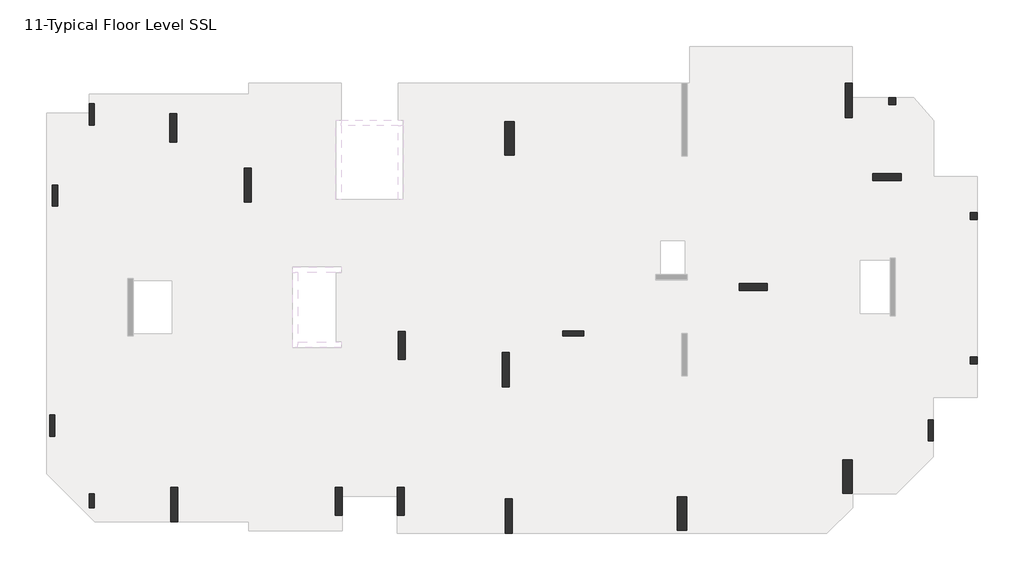
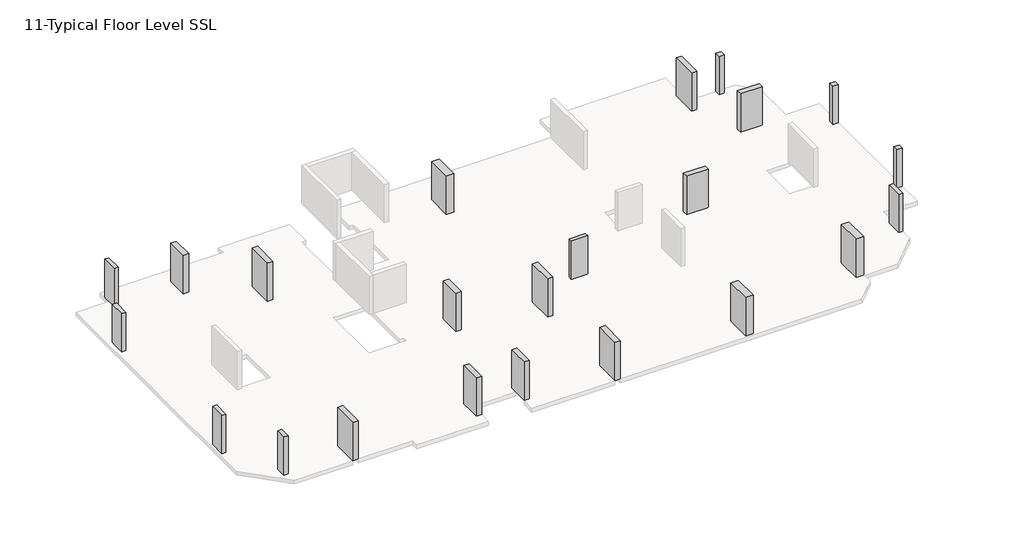
# One storey, part 2 of 2: 23 columns.
"""IFC4 building model written with IfcOpenShell, lengths in millimetres."""

import ifcopenshell
import ifcopenshell.guid

model = None  # the IFC model being written
_history = None  # IfcOwnerHistory: only IFC2X3 demands one
_inside = {}  # id of a spatial element -> (the spatial element, [elements in it])
_under = {}  # id of a project, library or spatial element -> (it, [spatial elements below it])
_declared = {}  # id of a project -> (the project, [libraries it declares])
_typed = {}  # id of a type object -> (the type object, [elements of that type])
_made_of = {}  # id of a material, layer set ... -> (it, [elements and type objects made of it])


def new_model(schema):
    """Start an empty IFC model of exactly this schema.

    Asked for "IFC4X3", IfcOpenShell would pick the latest addendum, in which some entities
    have other attributes; the version numbers below select the first issue.
    IFC2X3 requires an IfcOwnerHistory on every rooted entity: one is made here for all.
    """
    global model, _history
    if schema == "IFC4X3":
        model = ifcopenshell.file(schema_version=(4, 3, 0, 0))
    else:
        model = ifcopenshell.file(schema=schema)
    _inside.clear()
    _under.clear()
    _declared.clear()
    _typed.clear()
    _made_of.clear()
    _history = None
    if model.schema == "IFC2X3":
        org = make("IfcOrganization", Name="unknown")
        user = make(
            "IfcPersonAndOrganization",
            ThePerson=make("IfcPerson", FamilyName="unknown"),
            TheOrganization=org,
        )
        app = make(
            "IfcApplication",
            ApplicationDeveloper=org,
            Version="unknown",
            ApplicationFullName="unknown",
            ApplicationIdentifier="unknown",
        )
        _history = make(
            "IfcOwnerHistory",
            OwningUser=user,
            OwningApplication=app,
            ChangeAction="ADDED",
            CreationDate=0,
        )
    return model


def make(cls, **values):
    """One entity of the class cls with the attributes given. An attribute that is None is left unset."""
    return model.create_entity(
        cls, **{name: value for name, value in values.items() if value is not None}
    )


def rooted(cls, **values):
    """An entity with a GlobalId (a new one), such as an element, a storey or a relation."""
    return make(cls, GlobalId=ifcopenshell.guid.new(), OwnerHistory=_history, **values)


def si_unit(unit_type, name, prefix=None):
    """IfcSIUnit, for example si_unit("LENGTHUNIT", "METRE", prefix="MILLI")."""
    return make("IfcSIUnit", UnitType=unit_type, Prefix=prefix, Name=name)


def assignment(units):
    """IfcUnitAssignment: the units of a project."""
    return None if units is None else make("IfcUnitAssignment", Units=units)


def point(xyz):
    """IfcCartesianPoint."""
    return None if xyz is None else make("IfcCartesianPoint", Coordinates=xyz)


def direction(xyz):
    """IfcDirection."""
    return None if xyz is None else make("IfcDirection", DirectionRatios=xyz)


def frame(location, z_axis=None, x_axis=None):
    """IfcAxis2Placement3D, a coordinate frame: its origin and axes. An axis left out is left unset."""
    return make(
        "IfcAxis2Placement3D",
        Location=point(location),
        Axis=direction(z_axis),
        RefDirection=direction(x_axis),
    )


def origin():
    """The frame at (0, 0, 0) with its axes left unset."""
    return frame((0.0, 0.0, 0.0))


def place(relative_to, where):
    """IfcLocalPlacement: puts the frame where relative to a parent placement (None: the world)."""
    return make(
        "IfcLocalPlacement", PlacementRelTo=relative_to, RelativePlacement=where
    )


def context(
    kind, dimensions, precision=None, world=None, true_north=None, identifier=None
):
    """IfcGeometricRepresentationContext, for example the 3D "Model" context."""
    return make(
        "IfcGeometricRepresentationContext",
        ContextIdentifier=identifier,
        ContextType=kind,
        CoordinateSpaceDimension=dimensions,
        Precision=precision,
        WorldCoordinateSystem=world,
        TrueNorth=true_north,
    )


def project(units=None, contexts=None):
    """IfcProject with its units and contexts."""
    return rooted(
        "IfcProject",
        Name="project",
        RepresentationContexts=contexts,
        UnitsInContext=assignment(units),
    )


def spatial(cls, under=None, at=None, **own):
    """A site, building, storey or space (cls), placed at a placement, below another one or the project."""
    s = rooted(cls, ObjectPlacement=at, **own)
    if under is not None:
        _under.setdefault(under.id(), (under, []))[1].append(s)
    return s


def faces_of(points, faces, orient=None, outer=None):
    """IfcFace entities. A face is a list of loops; a loop is a list of indices into points, from 0.

    orient and outer hold one flag for each loop. By default every Orientation is true, the
    first loop of a face is its IfcFaceOuterBound and the others are IfcFaceBound.
    """
    made = []
    for i, loops in enumerate(faces):
        bounds = []
        for j, loop in enumerate(loops):
            is_outer = j == 0 if outer is None else outer[i][j]
            bounds.append(
                make(
                    "IfcFaceOuterBound" if is_outer else "IfcFaceBound",
                    Bound=make("IfcPolyLoop", Polygon=[points[k] for k in loop]),
                    Orientation=True if orient is None else orient[i][j],
                )
            )
        made.append(make("IfcFace", Bounds=bounds))
    return made


def faceted_brep(points, faces, orient=None, outer=None, voids=None):
    """IfcFacetedBrep: a solid bounded by flat faces; with voids (closed shells), ...WithVoids."""
    shared = [point(p) for p in points]
    hull = make("IfcClosedShell", CfsFaces=faces_of(shared, faces, orient, outer))
    if voids is None:
        return make("IfcFacetedBrep", Outer=hull)
    return make(
        "IfcFacetedBrepWithVoids",
        Outer=hull,
        Voids=[
            make(cls, CfsFaces=faces_of(shared, fs, o, b)) for cls, fs, o, b in voids
        ],
    )


def shape(context_of_items, identifier, shape_type, items):
    """IfcShapeRepresentation: the items that make up one representation, for example the "Body"."""
    return make(
        "IfcShapeRepresentation",
        ContextOfItems=context_of_items,
        RepresentationIdentifier=identifier,
        RepresentationType=shape_type,
        Items=items,
    )


def made_of(thing, what):
    """Note that an element or type object is made of a material, layer set ...; save() writes the relation."""
    if what is not None:
        _made_of.setdefault(what.id(), (what, []))[1].append(thing)
    return thing


def element(
    cls,
    number,
    at=None,
    inside=None,
    cuts=None,
    type_object=None,
    material=None,
    context=None,
    identifier="Body",
    shape_type=None,
    held_by="IfcProductDefinitionShape",
    body=None,
    shapes=None,
    **own,
):
    """One element of the class cls, such as IfcWall. Its Tag is "e" and its number.

    at: its placement. inside: the storey or other place that contains it. cuts: it is an
    opening in that element (IfcRelVoidsElement). A single representation is given by context,
    identifier, shape_type and body (its items); several are given by shapes. held_by: the class
    of the entity that holds the representations. save() writes the other relations.
    """
    e = rooted(cls, Tag="e%d" % number, ObjectPlacement=at, **own)
    if body is not None:
        shapes = [shape(context, identifier, shape_type, body)]
    if shapes is not None:
        e.Representation = make(held_by, Representations=shapes)
    if inside is not None:
        _inside.setdefault(inside.id(), (inside, []))[1].append(e)
    if cuts is not None:
        rooted(
            "IfcRelVoidsElement", RelatingBuildingElement=cuts, RelatedOpeningElement=e
        )
    if type_object is not None:
        _typed.setdefault(type_object.id(), (type_object, []))[1].append(e)
    return made_of(e, material)


def aggregate(whole, parts):
    """IfcRelAggregates: a whole, such as a stair, and the parts it consists of."""
    return rooted("IfcRelAggregates", RelatingObject=whole, RelatedObjects=parts)


def save(model, path):
    """Write the relations noted so far, then the file.

    IfcRelAggregates (storeys below a building ...), IfcRelContainedInSpatialStructure (elements
    in a storey), IfcRelDefinesByType, IfcRelAssociatesMaterial and IfcRelDeclares: one each for
    every whole, place, type object, material and project.
    """
    for whole, parts in _under.values():
        aggregate(whole, parts)
    for where, things in _inside.values():
        rooted(
            "IfcRelContainedInSpatialStructure",
            RelatedElements=things,
            RelatingStructure=where,
        )
    for kind, things in _typed.values():
        rooted("IfcRelDefinesByType", RelatedObjects=things, RelatingType=kind)
    for what, things in _made_of.values():
        rooted("IfcRelAssociatesMaterial", RelatedObjects=things, RelatingMaterial=what)
    for by, libraries in _declared.values():
        rooted("IfcRelDeclares", RelatingContext=by, RelatedDefinitions=libraries)
    model.write(path)


model = new_model("IFC4")

# Units and contexts
model_context = context("Model", 3, world=origin())
ifc_project = project(units=[si_unit("LENGTHUNIT", "METRE", prefix="MILLI")], contexts=[model_context])

# Site, building, storey
site = spatial("IfcSite", under=ifc_project)
building = spatial("IfcBuilding", under=site)
storey = spatial("IfcBuildingStorey", under=building, Name="11-Typical Floor Level SSL", Elevation=27000.0)

# Columns
placement = place(None, origin())
element("IfcColumn", 1, ObjectType="M_Concrete-Rectangular-Column : C-1 (400 x 400mm)", at=placement, inside=storey, context=model_context, shape_type="Brep", body=[
    faceted_brep([(52549.9999998, 16712.0, 27000.0), (52549.9999998, 16312.0, 27000.0), (52149.9999998, 16312.0, 27000.0), (52149.9999998, 16712.0, 27000.0), (52549.9999998, 16712.0, 30000.0), (52549.9999998, 16312.0, 30000.0), (52549.9999998, 16312.0, 29700.0), (52549.9999998, 16712.0, 29700.0), (52149.9999998, 16312.0, 30000.0), (52149.9999998, 16312.0, 29700.0), (52149.9999998, 16712.0, 30000.0), (52149.9999998, 16712.0, 29700.0)], [[[0, 1, 2, 3]], [[4, 5, 6, 1, 0, 7]], [[5, 8, 9, 2, 1, 6]], [[8, 10, 11, 3, 2, 9]], [[10, 4, 7, 0, 3, 11]], [[4, 10, 8, 5]]]),
])
element("IfcColumn", 2, ObjectType="M_Concrete-Rectangular-Column : C-1 (400 x 400mm)", at=placement, inside=storey, context=model_context, shape_type="Brep", body=[
    faceted_brep([(47898.6337868, 23252.0, 27000.0), (47898.6337868, 22852.0, 27000.0), (47498.6337868, 22852.0, 27000.0), (47498.6337868, 23252.0, 27000.0), (47898.6337868, 23252.0, 30000.0), (47898.6337868, 22852.0, 30000.0), (47898.6337868, 22852.0, 29700.0), (47498.6337868, 22852.0, 30000.0), (47498.6337868, 22852.0, 29700.0), (47498.6337868, 23252.0, 30000.0)], [[[0, 1, 2, 3]], [[4, 5, 6, 1, 0]], [[5, 7, 8, 2, 1, 6]], [[7, 9, 3, 2, 8]], [[9, 4, 0, 3]], [[4, 9, 7, 5]]]),
])
element("IfcColumn", 3, ObjectType="M_Concrete-Rectangular-Column : C-1 (400 x 400mm)", at=placement, inside=storey, context=model_context, shape_type="Brep", body=[
    faceted_brep([(52549.9999998, 8504.0039609, 27000.0), (52549.9999998, 8104.0039609, 27000.0), (52149.9999998, 8104.0039609, 27000.0), (52149.9999998, 8504.0039609, 27000.0), (52549.9999998, 8504.0039609, 30000.0), (52549.9999998, 8104.0039609, 30000.0), (52549.9999998, 8104.0039609, 29700.0), (52549.9999998, 8504.0039609, 29700.0), (52149.9999998, 8104.0039609, 30000.0), (52149.9999998, 8104.0039609, 29700.0), (52149.9999998, 8504.0039609, 30000.0), (52149.9999998, 8504.0039609, 29700.0)], [[[0, 1, 2, 3]], [[4, 5, 6, 1, 0, 7]], [[5, 8, 9, 2, 1, 6]], [[8, 10, 11, 3, 2, 9]], [[10, 4, 7, 0, 3, 11]], [[4, 10, 8, 5]]]),
])
element("IfcColumn", 4, ObjectType="M_Concrete-Rectangular-Column : C-2 (300 x 800mm)", at=placement, inside=storey, context=model_context, shape_type="Brep", body=[
    faceted_brep([(2352.0, 728.0, 27000.0), (2352.0, -72.0, 27000.0), (2052.0, -72.0, 27000.0), (2052.0, 728.0, 27000.0), (2352.0, 728.0, 30000.0), (2352.0, -72.0, 30000.0), (2352.0, -72.0, 29700.0), (2352.0, 728.0, 29700.0), (2052.0, -72.0, 30000.0), (2052.0, -72.0, 29700.0), (2052.0, 728.0, 30000.0), (2052.0, 728.0, 29700.0)], [[[0, 1, 2, 3]], [[4, 5, 6, 1, 0, 7]], [[5, 8, 9, 2, 1, 6]], [[8, 10, 11, 3, 2, 9]], [[10, 4, 7, 0, 3, 11]], [[4, 10, 8, 5]]]),
])
element("IfcColumn", 5, ObjectType="M_Concrete-Rectangular-Column : C-3(300 x 1200mm)", at=placement, inside=storey, context=model_context, shape_type="Brep", body=[
    faceted_brep([(2352.0, 22908.0000656, 27000.0), (2352.0, 21708.0000656, 27000.0), (2052.0, 21708.0000656, 27000.0), (2052.0, 22908.0000656, 27000.0), (2352.0, 22908.0000656, 30000.0), (2352.0, 21708.0000656, 30000.0), (2352.0, 21708.0000656, 29700.0), (2352.0, 22908.0000656, 29700.0), (2052.0, 21708.0000656, 30000.0), (2052.0, 21708.0000656, 29700.0), (2052.0, 22380.0004589, 30000.0), (2052.0, 22908.0000656, 30000.0), (2052.0, 22908.0000656, 29700.0)], [[[0, 1, 2, 3]], [[4, 5, 6, 1, 0, 7]], [[5, 8, 9, 2, 1, 6]], [[8, 10, 11, 12, 3, 2, 9]], [[11, 4, 7, 0, 3, 12]], [[4, 11, 10, 8, 5]]]),
])
element("IfcColumn", 6, ObjectType="M_Concrete-Rectangular-Column : C-3(300 x 1200mm)", at=placement, inside=storey, context=model_context, shape_type="Brep", body=[
    faceted_brep([(257.9999999, 18288.0, 27000.0), (257.9999999, 17088.0, 27000.0), (-42.0000001, 17088.0, 27000.0), (-42.0000001, 18288.0, 27000.0), (257.9999999, 18288.0, 30000.0), (257.9999999, 17088.0, 30000.0), (257.9999999, 17088.0, 29700.0), (257.9999999, 18288.0, 29700.0), (-42.0000001, 17088.0, 30000.0), (-42.0000001, 17088.0, 29700.0), (-42.0000001, 18288.0, 30000.0), (-42.0000001, 18288.0, 29700.0)], [[[0, 1, 2, 3]], [[4, 5, 6, 1, 0, 7]], [[5, 8, 9, 2, 1, 6]], [[8, 10, 11, 3, 2, 9]], [[10, 4, 7, 0, 3, 11]], [[4, 10, 8, 5]]]),
])
element("IfcColumn", 7, ObjectType="M_Concrete-Rectangular-Column : C-3(300 x 1200mm)", at=placement, inside=storey, context=model_context, shape_type="Brep", body=[
    faceted_brep([(108.001803, 5201.9999858, 27000.0), (108.001803, 4001.9999858, 27000.0), (-191.998197, 4001.9999858, 27000.0), (-191.998197, 5201.9999858, 27000.0), (108.001803, 5201.9999858, 30000.0), (108.001803, 4001.9999858, 30000.0), (108.001803, 4001.9999858, 29700.0), (108.001803, 5201.9999858, 29700.0), (-191.998197, 4001.9999858, 30000.0), (-191.998197, 4001.9999858, 29700.0), (-191.998197, 5201.9999858, 30000.0), (-191.998197, 5201.9999858, 29700.0)], [[[0, 1, 2, 3]], [[4, 5, 6, 1, 0, 7]], [[5, 8, 9, 2, 1, 6]], [[8, 10, 11, 3, 2, 9]], [[10, 4, 7, 0, 3, 11]], [[4, 10, 8, 5]]]),
])
element("IfcColumn", 8, ObjectType="M_Concrete-Rectangular-Column : C-3(300 x 1200mm)", at=placement, inside=storey, context=model_context, shape_type="Brep", body=[
    faceted_brep([(50046.0009271, 4931.9999929, 27000.0), (50046.0009271, 3731.9999929, 27000.0), (49746.0009271, 3731.9999929, 27000.0), (49746.0009271, 4931.9999929, 27000.0), (50046.0009271, 4931.9999929, 30000.0), (50046.0009271, 3731.9999929, 30000.0), (50046.0009271, 3731.9999929, 29700.0), (50046.0009271, 4931.9999929, 29700.0), (49746.0009271, 3731.9999929, 30000.0), (49746.0009271, 3731.9999929, 29700.0), (49746.0009271, 4931.9999929, 30000.0), (49746.0009271, 4931.9999929, 29700.0)], [[[0, 1, 2, 3]], [[4, 5, 6, 1, 0, 7]], [[5, 8, 9, 2, 1, 6]], [[8, 10, 11, 3, 2, 9]], [[10, 4, 7, 0, 3, 11]], [[4, 10, 8, 5]]]),
])
element("IfcColumn", 9, ObjectType="M_Concrete-Rectangular-Column : C-3(300 x 1200mm)", at=placement, inside=storey, context=model_context, shape_type="Brep", body=[
    faceted_brep([(28975.9999998, 9996.0000019, 27000.0), (30175.9999998, 9996.0000019, 27000.0), (30175.9999998, 9696.0000019, 27000.0), (28975.9999998, 9696.0000019, 27000.0), (28975.9999998, 9996.0000019, 30000.0), (30175.9999998, 9996.0000019, 30000.0), (30175.9999998, 9996.0000019, 29700.0), (28975.9999998, 9996.0000019, 29700.0), (30175.9999998, 9696.0000019, 30000.0), (30175.9999998, 9696.0000019, 29700.0), (28975.9999998, 9696.0000019, 30000.0), (28975.9999998, 9696.0000019, 29700.0)], [[[0, 1, 2, 3]], [[4, 5, 6, 1, 0, 7]], [[5, 8, 9, 2, 1, 6]], [[8, 10, 11, 3, 2, 9]], [[10, 4, 7, 0, 3, 11]], [[4, 10, 8, 5]]]),
])
element("IfcColumn", 10, ObjectType="M_Concrete-Rectangular-Column : C-4 (400 x 1600mm)", at=placement, inside=storey, context=model_context, shape_type="Brep", body=[
    faceted_brep([(7021.9999999, 22340.0000078, 27000.0), (7021.9999999, 20740.0000078, 27000.0), (6621.9999999, 20740.0000078, 27000.0), (6621.9999999, 22340.0000078, 27000.0), (7021.9999999, 22340.0000078, 30000.0), (7021.9999999, 20740.0000078, 30000.0), (7021.9999999, 20740.0000078, 29700.0), (7021.9999999, 22340.0000078, 29700.0), (6621.9999999, 20740.0000078, 30000.0), (6621.9999999, 20740.0000078, 29700.0), (6621.9999999, 22340.0000078, 30000.0), (6621.9999999, 22340.0000078, 29700.0)], [[[0, 1, 2, 3]], [[4, 5, 6, 1, 0, 7]], [[5, 8, 9, 2, 1, 6]], [[8, 10, 11, 3, 2, 9]], [[10, 4, 7, 0, 3, 11]], [[4, 10, 8, 5]]]),
])
element("IfcColumn", 11, ObjectType="M_Concrete-Rectangular-Column : C-4 (400 x 1600mm)", at=placement, inside=storey, context=model_context, shape_type="Brep", body=[
    faceted_brep([(19969.9997488, 1087.9955348, 27000.0), (19969.9997488, -512.0044652, 27000.0), (19569.9997488, -512.0044652, 27000.0), (19569.9997488, 1087.9955348, 27000.0), (19969.9997488, 1087.9955348, 30000.0), (19969.9997488, -512.0044652, 30000.0), (19969.9997488, -512.0044652, 29700.0), (19969.9997488, 1087.9955348, 29700.0), (19569.9997488, -512.0044652, 30000.0), (19569.9997488, -512.0044652, 29700.0), (19569.9997488, 564.000519, 30000.0), (19569.9997488, 1087.9955348, 30000.0), (19569.9997488, 1087.9955348, 29700.0)], [[[0, 1, 2, 3]], [[4, 5, 6, 1, 0, 7]], [[5, 8, 9, 2, 1, 6]], [[8, 10, 11, 12, 3, 2, 9]], [[11, 4, 7, 0, 3, 12]], [[4, 11, 10, 8, 5]]]),
])
element("IfcColumn", 12, ObjectType="M_Concrete-Rectangular-Column : C-4 (400 x 1600mm)", at=placement, inside=storey, context=model_context, shape_type="Brep", body=[
    faceted_brep([(46605.9993605, 18950.0, 27000.0), (48205.9993605, 18950.0, 27000.0), (48205.9993605, 18550.0, 27000.0), (46605.9993605, 18550.0, 27000.0), (46605.9993605, 18950.0, 30000.0), (48205.9993605, 18950.0, 30000.0), (48205.9993605, 18950.0, 29700.0), (46605.9993605, 18950.0, 29700.0), (48205.9993605, 18550.0, 30000.0), (48205.9993605, 18550.0, 29700.0), (46605.9993605, 18550.0, 30000.0), (46605.9993605, 18550.0, 29700.0)], [[[0, 1, 2, 3]], [[4, 5, 6, 1, 0, 7]], [[5, 8, 9, 2, 1, 6]], [[8, 10, 11, 3, 2, 9]], [[10, 4, 7, 0, 3, 11]], [[4, 10, 8, 5]]]),
])
element("IfcColumn", 13, ObjectType="M_Concrete-Rectangular-Column : C-5 (400 x 1600mm)", at=placement, inside=storey, context=model_context, shape_type="Brep", body=[
    faceted_brep([(20030.000009, 9955.9999979, 27000.0), (20030.000009, 8355.9999979, 27000.0), (19630.000009, 8355.9999979, 27000.0), (19630.000009, 9955.9999979, 27000.0), (20030.000009, 9955.9999979, 30000.0), (20030.000009, 8355.9999979, 30000.0), (20030.000009, 8355.9999979, 29700.0), (20030.000009, 9955.9999979, 29700.0), (19630.000009, 8355.9999979, 30000.0), (19630.000009, 8355.9999979, 29700.0), (19630.000009, 9955.9999979, 30000.0), (19630.000009, 9955.9999979, 29700.0)], [[[0, 1, 2, 3]], [[4, 5, 6, 1, 0, 7]], [[5, 8, 9, 2, 1, 6]], [[8, 10, 11, 3, 2, 9]], [[10, 4, 7, 0, 3, 11]], [[4, 10, 8, 5]]]),
])
element("IfcColumn", 14, ObjectType="M_Concrete-Rectangular-Column : C-5 (400 x 1600mm)", at=placement, inside=storey, context=model_context, shape_type="Brep", body=[
    faceted_brep([(16429.9999981, 1088.0, 27000.0), (16429.9999981, -512.0, 27000.0), (16029.9999981, -512.0, 27000.0), (16029.9999981, 1088.0, 27000.0), (16429.9999981, 1088.0, 30000.0), (16429.9999981, 564.000519, 30000.0), (16429.9999981, -512.0, 30000.0), (16429.9999981, -512.0, 29700.0), (16429.9999981, 1088.0, 29700.0), (16029.9999981, -512.0, 30000.0), (16029.9999981, -512.0, 29700.0), (16029.9999981, 1088.0, 30000.0), (16029.9999981, 1088.0, 29700.0)], [[[0, 1, 2, 3]], [[4, 5, 6, 7, 1, 0, 8]], [[6, 9, 10, 2, 1, 7]], [[9, 11, 12, 3, 2, 10]], [[11, 4, 8, 0, 3, 12]], [[4, 11, 9, 6, 5]]]),
])
element("IfcColumn", 15, ObjectType="M_Concrete-Rectangular-Column : C-5 (400 x 1600mm)", at=placement, inside=storey, context=model_context, shape_type="Brep", body=[
    faceted_brep([(38998.0014887, 12692.0079212, 27000.0), (40598.0014887, 12692.0079212, 27000.0), (40598.0014887, 12292.0079212, 27000.0), (38998.0014887, 12292.0079212, 27000.0), (38998.0014887, 12692.0079212, 30000.0), (40598.0014887, 12692.0079212, 30000.0), (40598.0014887, 12692.0079212, 29700.0), (38998.0014887, 12692.0079212, 29700.0), (40598.0014887, 12292.0079212, 30000.0), (40598.0014887, 12292.0079212, 29700.0), (38998.0014887, 12292.0079212, 30000.0), (38998.0014887, 12292.0079212, 29700.0)], [[[0, 1, 2, 3]], [[4, 5, 6, 1, 0, 7]], [[5, 8, 9, 2, 1, 6]], [[8, 10, 11, 3, 2, 9]], [[10, 4, 7, 0, 3, 11]], [[4, 10, 8, 5]]]),
])
element("IfcColumn", 16, ObjectType="M_Concrete-Rectangular-Column : C-6 (400 x 1950mm)", at=placement, inside=storey, context=model_context, shape_type="Brep", body=[
    faceted_brep([(11270.0000427, 19262.9999996, 27000.0), (11270.0000427, 17312.9999996, 27000.0), (10870.0000427, 17312.9999996, 27000.0), (10870.0000427, 19262.9999996, 27000.0), (11270.0000427, 19262.9999996, 30000.0), (11270.0000427, 17312.9999996, 30000.0), (11270.0000427, 17312.9999996, 29700.0), (11270.0000427, 19262.9999996, 29700.0), (10870.0000427, 17312.9999996, 30000.0), (10870.0000427, 17312.9999996, 29700.0), (10870.0000427, 19262.9999996, 30000.0), (10870.0000427, 19262.9999996, 29700.0)], [[[0, 1, 2, 3]], [[4, 5, 6, 1, 0, 7]], [[5, 8, 9, 2, 1, 6]], [[8, 10, 11, 3, 2, 9]], [[10, 4, 7, 0, 3, 11]], [[4, 10, 8, 5]]]),
])
element("IfcColumn", 17, ObjectType="M_Concrete-Rectangular-Column : C-6 (400 x 1950mm)", at=placement, inside=storey, context=model_context, shape_type="Brep", body=[
    faceted_brep([(7082.0000416, 1083.0000153, 27000.0), (7082.0000416, -866.9999847, 27000.0), (6682.0000416, -866.9999847, 27000.0), (6682.0000416, 1083.0000153, 27000.0), (7082.0000416, 1083.0000153, 30000.0), (7082.0000416, -866.9999847, 30000.0), (7082.0000416, -866.9999847, 29700.0), (7082.0000416, 1083.0000153, 29700.0), (6682.0000416, -866.9999847, 30000.0), (6682.0000416, -866.9999847, 29700.0), (6682.0000416, 1083.0000153, 30000.0), (6682.0000416, 1083.0000153, 29700.0)], [[[0, 1, 2, 3]], [[4, 5, 6, 1, 0, 7]], [[5, 8, 9, 2, 1, 6]], [[8, 10, 11, 3, 2, 9]], [[10, 4, 7, 0, 3, 11]], [[4, 10, 8, 5]]]),
])
element("IfcColumn", 18, ObjectType="M_Concrete-Rectangular-Column : C-6 (400 x 1950mm)", at=placement, inside=storey, context=model_context, shape_type="Brep", body=[
    faceted_brep([(26113.9999998, 422.995535, 27000.0), (26113.9999998, -1527.004465, 27000.0), (25713.9999998, -1527.004465, 27000.0), (25713.9999998, 422.995535, 27000.0), (26113.9999998, 422.995535, 30000.0), (26113.9999998, -1527.004465, 30000.0), (26113.9999998, -1527.004465, 29700.0), (26113.9999998, 422.995535, 29700.0), (25713.9999998, -1527.004465, 30000.0), (25713.9999998, -1527.004465, 29700.0), (25713.9999998, 422.995535, 30000.0), (25713.9999998, 422.995535, 29700.0)], [[[0, 1, 2, 3]], [[4, 5, 6, 1, 0, 7]], [[5, 8, 9, 2, 1, 6]], [[8, 10, 11, 3, 2, 9]], [[10, 4, 7, 0, 3, 11]], [[4, 10, 8, 5]]]),
])
element("IfcColumn", 19, ObjectType="M_Concrete-Rectangular-Column : C-6 (400 x 1950mm)", at=placement, inside=storey, context=model_context, shape_type="Brep", body=[
    faceted_brep([(45446.0007483, 24087.0, 27000.0), (45446.0007483, 22137.0, 27000.0), (45046.0007483, 22137.0, 27000.0), (45046.0007483, 24087.0, 27000.0), (45446.0007483, 24087.0, 30000.0), (45446.0007483, 23252.0000315, 30000.0), (45446.0007483, 22137.0, 30000.0), (45446.0007483, 22137.0, 29700.0), (45446.0007483, 24087.0, 29700.0), (45046.0007483, 22137.0, 30000.0), (45046.0007483, 22137.0, 29700.0), (45046.0007483, 24087.0, 30000.0), (45046.0007483, 24087.0, 29700.0)], [[[0, 1, 2, 3]], [[4, 5, 6, 7, 1, 0, 8]], [[6, 9, 10, 2, 1, 7]], [[9, 11, 12, 3, 2, 10]], [[11, 4, 8, 0, 3, 12]], [[4, 11, 9, 6, 5]]]),
])
element("IfcColumn", 20, ObjectType="M_Concrete-Rectangular-Column : C-6 (400 x 1950mm)", at=placement, inside=storey, context=model_context, shape_type="Brep", body=[
    faceted_brep([(25934.0000455, 8751.0001824, 27000.0), (25934.0000455, 6801.0001824, 27000.0), (25534.0000455, 6801.0001824, 27000.0), (25534.0000455, 8751.0001824, 27000.0), (25934.0000455, 8751.0001824, 30000.0), (25934.0000455, 6801.0001824, 30000.0), (25934.0000455, 6801.0001824, 29700.0), (25934.0000455, 8751.0001824, 29700.0), (25534.0000455, 6801.0001824, 30000.0), (25534.0000455, 6801.0001824, 29700.0), (25534.0000455, 8751.0001824, 30000.0), (25534.0000455, 8751.0001824, 29700.0)], [[[0, 1, 2, 3]], [[4, 5, 6, 1, 0, 7]], [[5, 8, 9, 2, 1, 6]], [[8, 10, 11, 3, 2, 9]], [[10, 4, 7, 0, 3, 11]], [[4, 10, 8, 5]]]),
])
element("IfcColumn", 21, ObjectType="M_Concrete-Rectangular-Column : C-7 (550 x 1900mm)", at=placement, inside=storey, context=model_context, shape_type="Brep", body=[
    faceted_brep([(36035.9999998, 548.0007983, 27000.0), (36035.9999998, -1351.9992017, 27000.0), (35485.9999998, -1351.9992017, 27000.0), (35485.9999998, 548.0007983, 27000.0), (36035.9999998, 548.0007983, 30000.0), (36035.9999998, -1351.9992017, 30000.0), (36035.9999998, -1351.9992017, 29700.0), (36035.9999998, 548.0007983, 29700.0), (35485.9999998, -1351.9992017, 30000.0), (35485.9999998, -1351.9992017, 29700.0), (35485.9999998, 548.0007983, 30000.0), (35485.9999998, 548.0007983, 29700.0)], [[[0, 1, 2, 3]], [[4, 5, 6, 1, 0, 7]], [[5, 8, 9, 2, 1, 6]], [[8, 10, 11, 3, 2, 9]], [[10, 4, 7, 0, 3, 11]], [[4, 10, 8, 5]]]),
])
element("IfcColumn", 22, ObjectType="M_Concrete-Rectangular-Column : C-7 (550 x 1900mm)", at=placement, inside=storey, context=model_context, shape_type="Brep", body=[
    faceted_brep([(45443.9999998, 2648.0, 27000.0), (45443.9999998, 748.0, 27000.0), (44893.9999998, 748.0, 27000.0), (44893.9999998, 2648.0, 27000.0), (45443.9999998, 2648.0, 30000.0), (45443.9999998, 748.0, 30000.0), (45443.9999998, 748.0, 29700.0), (45443.9999998, 2648.0, 29700.0), (44893.9999998, 748.0, 30000.0), (44893.9999998, 748.0, 29700.0), (44893.9999998, 2648.0, 30000.0), (44893.9999998, 2648.0, 29700.0)], [[[0, 1, 2, 3]], [[4, 5, 6, 1, 0, 7]], [[5, 8, 9, 2, 1, 6]], [[8, 10, 11, 3, 2, 9]], [[10, 4, 7, 0, 3, 11]], [[4, 10, 8, 5]]]),
])
element("IfcColumn", 23, ObjectType="M_Concrete-Rectangular-Column : C-7 (550 x 1900mm)", at=placement, inside=storey, context=model_context, shape_type="Brep", body=[
    faceted_brep([(26218.9999998, 21900.0, 27000.0), (26218.9999998, 20000.0, 27000.0), (25668.9999998, 20000.0, 27000.0), (25668.9999998, 21900.0, 27000.0), (26218.9999998, 21900.0, 30000.0), (26218.9999998, 20000.0, 30000.0), (26218.9999998, 20000.0, 29700.0), (26218.9999998, 21900.0, 29700.0), (25668.9999998, 20000.0, 30000.0), (25668.9999998, 20000.0, 29700.0), (25668.9999998, 21900.0, 30000.0), (25668.9999998, 21900.0, 29700.0)], [[[0, 1, 2, 3]], [[4, 5, 6, 1, 0, 7]], [[5, 8, 9, 2, 1, 6]], [[8, 10, 11, 3, 2, 9]], [[10, 4, 7, 0, 3, 11]], [[4, 10, 8, 5]]]),
])

save(model, "model.ifc")

# Revit data of these elements
# Type "M_Concrete-Rectangular-Column : C-1 (400 x 400mm)"
#   Type Mark = "C01"
#   b = 400 mm
#   h = 400 mm
#   Structural Material [instance default] = Concrete, Cast-in-Place gray
# Type "M_Concrete-Rectangular-Column : C-2 (300 x 800mm)"
#   Type Mark = "C02"
#   b = 300 mm
#   h = 800 mm
#   Structural Material [instance default] = Concrete, Cast-in-Place gray
# Type "M_Concrete-Rectangular-Column : C-3(300 x 1200mm)"
#   Type Mark = "C03"
#   b = 300 mm
#   h = 1200 mm
#   Structural Material [instance default] = Concrete, Cast-in-Place gray
# Type "M_Concrete-Rectangular-Column : C-4 (400 x 1600mm)"
#   Type Mark = "C04"
#   b = 400 mm
#   h = 1600 mm
#   Structural Material [instance default] = Concrete, Cast-in-Place gray
# Type "M_Concrete-Rectangular-Column : C-5 (400 x 1600mm)"
#   Type Mark = "C05"
#   b = 400 mm
#   h = 1600 mm
#   Structural Material [instance default] = Concrete, Cast-in-Place gray
# Type "M_Concrete-Rectangular-Column : C-6 (400 x 1950mm)"
#   Type Mark = "C06"
#   b = 400 mm
#   h = 1950 mm
#   Structural Material [instance default] = Concrete, Cast-in-Place gray
# Type "M_Concrete-Rectangular-Column : C-7 (550 x 1900mm)"
#   Type Mark = "C07"
#   b = 550 mm
#   h = 1900 mm
#   Structural Material [instance default] = Concrete, Cast-in-Place gray
# Elements 1, 2, 3 (IfcColumn, "M_Concrete-Rectangular-Column : C-1 (400 x 400mm)")
#   Structural Material = Concrete-RC
#   Phase Created = New Construction
#   Materials on its faces: "Concrete-RC"
# Element 4 (IfcColumn, "M_Concrete-Rectangular-Column : C-2 (300 x 800mm)")
#   Structural Material = Concrete-RC
#   Phase Created = New Construction
#   Materials on its faces: "Concrete-RC"
# Elements 5, 6, 7, 8, 9 (IfcColumn, "M_Concrete-Rectangular-Column : C-3(300 x 1200mm)")
#   Structural Material = Concrete-RC
#   Phase Created = New Construction
#   Materials on its faces: "Concrete-RC"
# Elements 10, 11, 12 (IfcColumn, "M_Concrete-Rectangular-Column : C-4 (400 x 1600mm)")
#   Structural Material = Concrete-RC
#   Phase Created = New Construction
#   Materials on its faces: "Concrete-RC"
# Elements 13, 14, 15 (IfcColumn, "M_Concrete-Rectangular-Column : C-5 (400 x 1600mm)")
#   Structural Material = Concrete-RC
#   Phase Created = New Construction
#   Materials on its faces: "Concrete-RC"
# Elements 16, 17, 18, 19, 20 (IfcColumn, "M_Concrete-Rectangular-Column : C-6 (400 x 1950mm)")
#   Structural Material = Concrete-RC
#   Phase Created = New Construction
#   Materials on its faces: "Concrete-RC"
# Elements 21, 22, 23 (IfcColumn, "M_Concrete-Rectangular-Column : C-7 (550 x 1900mm)")
#   Structural Material = Concrete-RC
#   Phase Created = New Construction
#   Materials on its faces: "Concrete-RC"
# Materials
#   "Concrete, Cast-in-Place gray": class "Concrete", colour RGB 192 192 192, transparency 0, Description = "Cast-in-place concrete", Cost = 0
#   "Concrete-RC": class "Concrete", colour RGB 128 128 128, transparency 0, Description = "High strength concrete", Cost = 0
